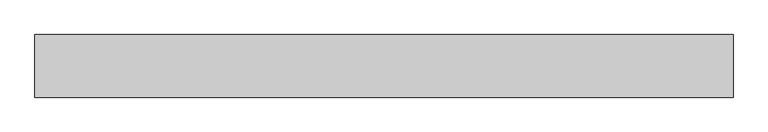
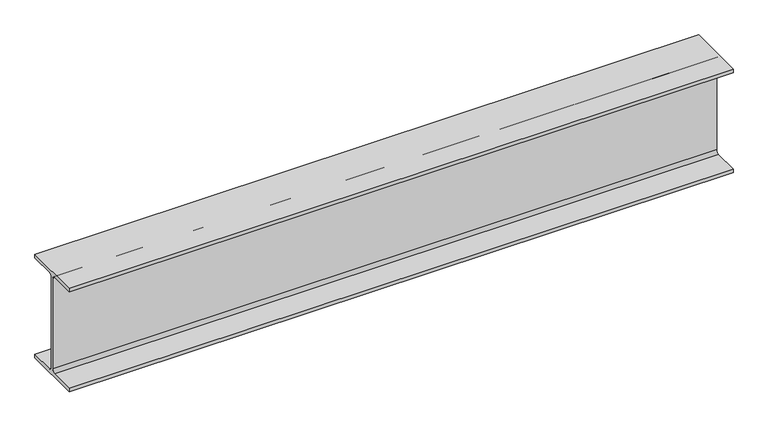
"""IFC4 building model written with IfcOpenShell, lengths in millimetres: beam geometry, Old_Steel Beam_H-KSD3502 : H_SB_ASB_H-194×150x6x9."""

import ifcopenshell
import ifcopenshell.guid

model = None  # the IFC model being written
_history = None  # IfcOwnerHistory: only IFC2X3 demands one
_inside = {}  # id of a spatial element -> (the spatial element, [elements in it])
_under = {}  # id of a project, library or spatial element -> (it, [spatial elements below it])
_declared = {}  # id of a project -> (the project, [libraries it declares])
_typed = {}  # id of a type object -> (the type object, [elements of that type])
_made_of = {}  # id of a material, layer set ... -> (it, [elements and type objects made of it])


def new_model(schema):
    """Start an empty IFC model of exactly this schema.

    Asked for "IFC4X3", IfcOpenShell would pick the latest addendum, in which some entities
    have other attributes; the version numbers below select the first issue.
    IFC2X3 requires an IfcOwnerHistory on every rooted entity: one is made here for all.
    """
    global model, _history
    if schema == "IFC4X3":
        model = ifcopenshell.file(schema_version=(4, 3, 0, 0))
    else:
        model = ifcopenshell.file(schema=schema)
    _inside.clear()
    _under.clear()
    _declared.clear()
    _typed.clear()
    _made_of.clear()
    _history = None
    if model.schema == "IFC2X3":
        org = make("IfcOrganization", Name="unknown")
        user = make(
            "IfcPersonAndOrganization",
            ThePerson=make("IfcPerson", FamilyName="unknown"),
            TheOrganization=org,
        )
        app = make(
            "IfcApplication",
            ApplicationDeveloper=org,
            Version="unknown",
            ApplicationFullName="unknown",
            ApplicationIdentifier="unknown",
        )
        _history = make(
            "IfcOwnerHistory",
            OwningUser=user,
            OwningApplication=app,
            ChangeAction="ADDED",
            CreationDate=0,
        )
    return model


def make(cls, **values):
    """One entity of the class cls with the attributes given. An attribute that is None is left unset."""
    return model.create_entity(
        cls, **{name: value for name, value in values.items() if value is not None}
    )


def rooted(cls, **values):
    """An entity with a GlobalId (a new one), such as an element, a storey or a relation."""
    return make(cls, GlobalId=ifcopenshell.guid.new(), OwnerHistory=_history, **values)


def si_unit(unit_type, name, prefix=None):
    """IfcSIUnit, for example si_unit("LENGTHUNIT", "METRE", prefix="MILLI")."""
    return make("IfcSIUnit", UnitType=unit_type, Prefix=prefix, Name=name)


def assignment(units):
    """IfcUnitAssignment: the units of a project."""
    return None if units is None else make("IfcUnitAssignment", Units=units)


def point(xyz):
    """IfcCartesianPoint."""
    return None if xyz is None else make("IfcCartesianPoint", Coordinates=xyz)


def direction(xyz):
    """IfcDirection."""
    return None if xyz is None else make("IfcDirection", DirectionRatios=xyz)


def frame(location, z_axis=None, x_axis=None):
    """IfcAxis2Placement3D, a coordinate frame: its origin and axes. An axis left out is left unset."""
    return make(
        "IfcAxis2Placement3D",
        Location=point(location),
        Axis=direction(z_axis),
        RefDirection=direction(x_axis),
    )


def frame_2d(location, x_axis=None):
    """IfcAxis2Placement2D, a coordinate frame in the plane: its origin and x axis."""
    return make(
        "IfcAxis2Placement2D", Location=point(location), RefDirection=direction(x_axis)
    )


def origin():
    """The frame at (0, 0, 0) with its axes left unset."""
    return frame((0.0, 0.0, 0.0))


def place(relative_to, where):
    """IfcLocalPlacement: puts the frame where relative to a parent placement (None: the world)."""
    return make(
        "IfcLocalPlacement", PlacementRelTo=relative_to, RelativePlacement=where
    )


def context(
    kind, dimensions, precision=None, world=None, true_north=None, identifier=None
):
    """IfcGeometricRepresentationContext, for example the 3D "Model" context."""
    return make(
        "IfcGeometricRepresentationContext",
        ContextIdentifier=identifier,
        ContextType=kind,
        CoordinateSpaceDimension=dimensions,
        Precision=precision,
        WorldCoordinateSystem=world,
        TrueNorth=true_north,
    )


def project(units=None, contexts=None):
    """IfcProject with its units and contexts."""
    return rooted(
        "IfcProject",
        Name="project",
        RepresentationContexts=contexts,
        UnitsInContext=assignment(units),
    )


def spatial(cls, under=None, at=None, **own):
    """A site, building, storey or space (cls), placed at a placement, below another one or the project."""
    s = rooted(cls, ObjectPlacement=at, **own)
    if under is not None:
        _under.setdefault(under.id(), (under, []))[1].append(s)
    return s


def polyline(points):
    """IfcPolyline through the points."""
    return make("IfcPolyline", Points=[point(p) for p in points])


def circle_curve(where, radius):
    """IfcCircle in the frame where."""
    return make("IfcCircle", Position=where, Radius=radius)


def trimmed(basis, trim1, trim2, sense, master):
    """IfcTrimmedCurve: the piece of a basis curve between two trims."""
    return make(
        "IfcTrimmedCurve",
        BasisCurve=basis,
        Trim1=trim1,
        Trim2=trim2,
        SenseAgreement=sense,
        MasterRepresentation=master,
    )


def segment(curve, same_sense, transition):
    """IfcCompositeCurveSegment."""
    return make(
        "IfcCompositeCurveSegment",
        Transition=transition,
        SameSense=same_sense,
        ParentCurve=curve,
    )


def composite_curve(segments, self_intersect=None):
    """IfcCompositeCurve: segments joined end to end."""
    return make("IfcCompositeCurve", Segments=segments, SelfIntersect=self_intersect)


def outline(outer, holes=None, kind="AREA"):
    """IfcArbitraryClosedProfileDef: a profile drawn as a closed curve; with holes, ...WithVoids."""
    if holes is None:
        return make("IfcArbitraryClosedProfileDef", ProfileType=kind, OuterCurve=outer)
    return make(
        "IfcArbitraryProfileDefWithVoids",
        ProfileType=kind,
        OuterCurve=outer,
        InnerCurves=holes,
    )


def extrude(swept, where, along, depth):
    """IfcExtrudedAreaSolid: the profile swept, set in the frame where, extruded along a direction by depth."""
    return make(
        "IfcExtrudedAreaSolid",
        SweptArea=swept,
        Position=where,
        ExtrudedDirection=direction(along),
        Depth=depth,
    )


def shape(context_of_items, identifier, shape_type, items):
    """IfcShapeRepresentation: the items that make up one representation, for example the "Body"."""
    return make(
        "IfcShapeRepresentation",
        ContextOfItems=context_of_items,
        RepresentationIdentifier=identifier,
        RepresentationType=shape_type,
        Items=items,
    )


def source(mapping_origin, context_of_items, identifier, shape_type, items):
    """IfcRepresentationMap: a shape defined once, which mapped items show again and again."""
    return make(
        "IfcRepresentationMap",
        MappingOrigin=mapping_origin,
        MappedRepresentation=shape(context_of_items, identifier, shape_type, items),
    )


def transform(
    local_origin,
    x_axis=None,
    y_axis=None,
    z_axis=None,
    scale=None,
    scale2=None,
    scale3=None,
    uniform=True,
):
    """IfcCartesianTransformationOperator3D, or its non-uniform kind. x_axis, y_axis, z_axis: its Axis1, 2, 3."""
    if uniform:
        return make(
            "IfcCartesianTransformationOperator3D",
            Axis1=direction(x_axis),
            Axis2=direction(y_axis),
            LocalOrigin=point(local_origin),
            Scale=scale,
            Axis3=direction(z_axis),
        )
    return make(
        "IfcCartesianTransformationOperator3DnonUniform",
        Axis1=direction(x_axis),
        Axis2=direction(y_axis),
        LocalOrigin=point(local_origin),
        Scale=scale,
        Axis3=direction(z_axis),
        Scale2=scale2,
        Scale3=scale3,
    )


def mapped(mapping_source, mapping_target):
    """IfcMappedItem: shows the shape of a source again, moved by a transform."""
    return make(
        "IfcMappedItem", MappingSource=mapping_source, MappingTarget=mapping_target
    )


def made_of(thing, what):
    """Note that an element or type object is made of a material, layer set ...; save() writes the relation."""
    if what is not None:
        _made_of.setdefault(what.id(), (what, []))[1].append(thing)
    return thing


def element(
    cls,
    number,
    at=None,
    inside=None,
    cuts=None,
    type_object=None,
    material=None,
    context=None,
    identifier="Body",
    shape_type=None,
    held_by="IfcProductDefinitionShape",
    body=None,
    shapes=None,
    **own,
):
    """One element of the class cls, such as IfcWall. Its Tag is "e" and its number.

    at: its placement. inside: the storey or other place that contains it. cuts: it is an
    opening in that element (IfcRelVoidsElement). A single representation is given by context,
    identifier, shape_type and body (its items); several are given by shapes. held_by: the class
    of the entity that holds the representations. save() writes the other relations.
    """
    e = rooted(cls, Tag="e%d" % number, ObjectPlacement=at, **own)
    if body is not None:
        shapes = [shape(context, identifier, shape_type, body)]
    if shapes is not None:
        e.Representation = make(held_by, Representations=shapes)
    if inside is not None:
        _inside.setdefault(inside.id(), (inside, []))[1].append(e)
    if cuts is not None:
        rooted(
            "IfcRelVoidsElement", RelatingBuildingElement=cuts, RelatedOpeningElement=e
        )
    if type_object is not None:
        _typed.setdefault(type_object.id(), (type_object, []))[1].append(e)
    return made_of(e, material)


def aggregate(whole, parts):
    """IfcRelAggregates: a whole, such as a stair, and the parts it consists of."""
    return rooted("IfcRelAggregates", RelatingObject=whole, RelatedObjects=parts)


def save(model, path):
    """Write the relations noted so far, then the file.

    IfcRelAggregates (storeys below a building ...), IfcRelContainedInSpatialStructure (elements
    in a storey), IfcRelDefinesByType, IfcRelAssociatesMaterial and IfcRelDeclares: one each for
    every whole, place, type object, material and project.
    """
    for whole, parts in _under.values():
        aggregate(whole, parts)
    for where, things in _inside.values():
        rooted(
            "IfcRelContainedInSpatialStructure",
            RelatedElements=things,
            RelatingStructure=where,
        )
    for kind, things in _typed.values():
        rooted("IfcRelDefinesByType", RelatedObjects=things, RelatingType=kind)
    for what, things in _made_of.values():
        rooted("IfcRelAssociatesMaterial", RelatedObjects=things, RelatingMaterial=what)
    for by, libraries in _declared.values():
        rooted("IfcRelDeclares", RelatingContext=by, RelatedDefinitions=libraries)
    model.write(path)


def beam_91d8de06(model_context):
    return source(origin(), model_context, "Body", "SweptSolid", [
        extrude(outline(composite_curve([segment(polyline([(-82.5, -141.5), (-11.9, -141.5)]), True, "CONTINUOUS"), segment(trimmed(circle_curve(frame_2d((-11.9, -132.6)), 8.9), [point((-11.9, -141.5))], [point((-3.0, -132.6))], True, "CARTESIAN"), True, "CONTINUOUS"), segment(polyline([(-3.0, -132.6), (-3.0, 132.6)]), True, "CONTINUOUS"), segment(trimmed(circle_curve(frame_2d((-11.9, 132.6)), 8.9), [point((-3.0, 132.6))], [point((-11.9, 141.5))], True, "CARTESIAN"), True, "CONTINUOUS"), segment(polyline([(-11.9, 141.5), (-82.5, 141.5), (-82.5, 151.7), (82.5, 151.7), (82.5, 141.5), (11.9, 141.5)]), True, "CONTINUOUS"), segment(trimmed(circle_curve(frame_2d((11.9, 132.6)), 8.9), [point((11.9, 141.5))], [point((3.0, 132.6))], True, "CARTESIAN"), True, "CONTINUOUS"), segment(polyline([(3.0, 132.6), (3.0, -132.6)]), True, "CONTINUOUS"), segment(trimmed(circle_curve(frame_2d((11.9, -132.6)), 8.9), [point((3.0, -132.6))], [point((11.9, -141.5))], True, "CARTESIAN"), True, "CONTINUOUS"), segment(polyline([(11.9, -141.5), (82.5, -141.5), (82.5, -151.7), (-82.5, -151.7), (-82.5, -141.5)]), True, "CONTINUOUS")], self_intersect=False)), frame((-851.3274068, 0.0, 0.0), z_axis=(1.0, 0.0, 0.0), x_axis=(0.0, 1.0, 0.0)), (0.0, 0.0, 1.0), 1839.6820153),
    ])


if __name__ == "__main__":
    model = new_model("IFC4")
    model_context = context("Model", 3, world=origin())
    ifc_project = project(units=[si_unit("LENGTHUNIT", "METRE", prefix="MILLI")], contexts=[model_context])
    site = spatial("IfcSite", under=ifc_project)
    building = spatial("IfcBuilding", under=site)
    placement = place(None, origin())
    beam_shape = beam_91d8de06(model_context)
    element("IfcBeam", 1, ObjectType="Old_Steel Beam_H-KSD3502 : H_SB_ASB_H-194×150x6x9", at=placement, inside=building, context=model_context, shape_type="MappedRepresentation", body=[
        mapped(beam_shape, transform((0.0, 0.0, 0.0), x_axis=(1.0, 0.0, 0.0), y_axis=(0.0, 1.0, 0.0), z_axis=(0.0, 0.0, 1.0))),
    ])
    save(model, "model.ifc")

# Revit data of these elements
# Type "Old_Steel Beam_H-KSD3502 : H_SB_ASB_H-194×150x6x9"
#   Width = 15.0 cm
#   Web Thickness = 0.6 cm
#   Web Fillet = 1.3 cm
#   Warping Constant = 43316.0 cm⁶
#   Torsional Moment of Inertia = 8.622 cm⁴
#   Torsional Modulus = 1.0 cm³
#   Section Area = 39.01 cm²
#   Plastic Modulus weak axis = 104.0 cm³
#   Plastic Modulus strong axis = 309.0 cm³
#   Perimeter = 0.95 m²/m
#   Nominal Weight = 30.60 kgf/m
#   Moment of Inertia weak axis = 507.00 cm⁴
#   Moment of Inertia strong axis = 2690.00 cm⁴
#   Height = 19.4 cm
#   Flange Thickness = 0.9 cm
#   Elastic Modulus weak axis = 67.6 cm³
#   Elastic Modulus strong axis = 277.0 cm³
#   Centroid Vertical = 9.7 cm
#   Centroid Horizontal = 7.5 cm
#   Length [instance default] = 1.5240 m
#   Structural Material [instance default] = Steel, 45-345
#   Assembly Code = ""
# Element 1 (IfcBeam, "Old_Steel Beam_H-KSD3502 : H_SB_ASB_H-194×150x6x9")
#   Structural Material = none
# Materials
#   "Steel, 45-345": class "Metal", colour RGB 189 187 185, transparency 0, Description = "Steel 345 MPa", Cost = 0
